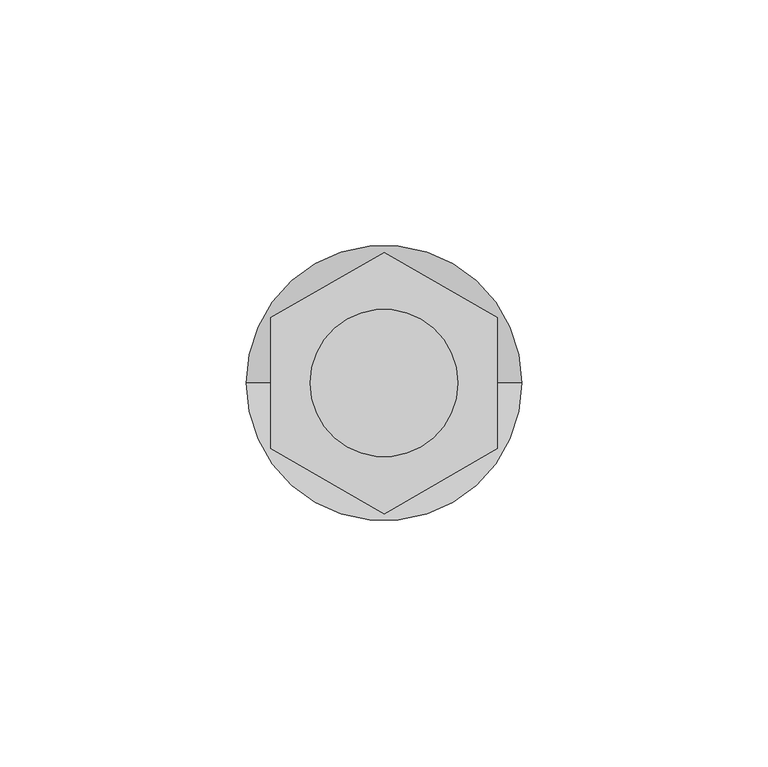
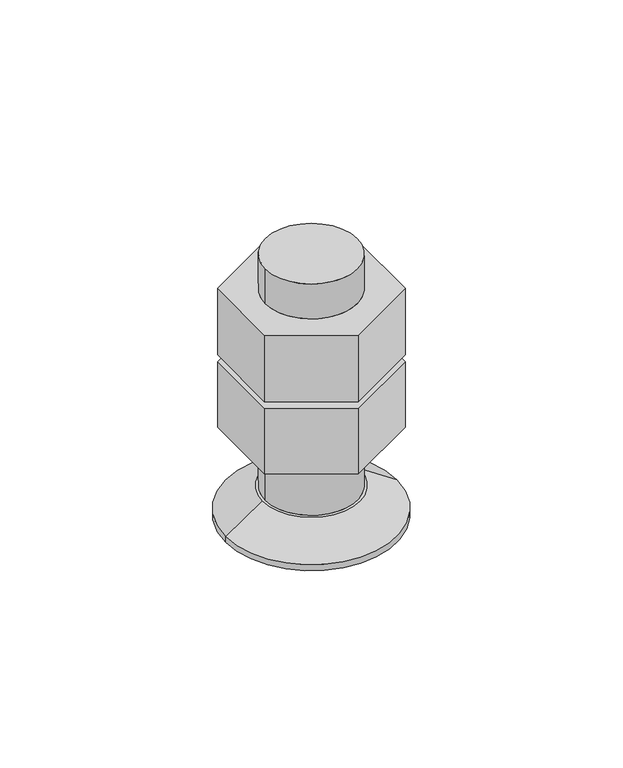
"""IFC4 building model written with IfcOpenShell, lengths in millimetres: fastener geometry, Bolt HPM-L : 30/L_mk."""

from ifc_helpers import new_model, si_unit, frame, origin, origin_with_axes, place, context, project, spatial, polyline, circle_curve, source, transform, mapped, element, save
from ifc_brep_helpers import plane_surface, cylinder_surface, revolved_surface, advanced_brep


def fastener_4f65ad77(model_context):
    return source(origin(), model_context, "Body", "AdvancedBrep", [
        advanced_brep(
        [(-23.0, 13.2790562, 22.7), (-23.0, -13.2790562, 22.7), (0.0, -26.5581124, 22.7), (23.0, -13.2790562, 22.7), (23.0, 13.2790562, 22.7), (0.0, 26.5581124, 22.7), (15.0, 0.0, 22.7), (-15.0, 0.0, 22.7), (-23.0, 13.2790562, 0.0), (0.0, 26.5581124, 0.0), (23.0, 13.2790562, 0.0), (23.0, -13.2790562, 0.0), (0.0, -26.5581124, 0.0), (-23.0, -13.2790562, 0.0), (-15.0, 0.0, 0.0), (15.0, 0.0, 0.0), (-15.0, 0.0, 60.0), (15.0, 0.0, 60.0), (15.0, 0.0, 25.0), (-15.0, 0.0, 25.0), (-15.0, 0.0, 48.0), (15.0, 0.0, 48.0), (-15.0, 0.0, -20.0), (15.0, 0.0, -20.0), (-23.0, 13.2790562, 48.0), (-23.0, -13.2790562, 48.0), (0.0, -26.5581124, 48.0), (23.0, -13.2790562, 48.0), (23.0, 13.2790562, 48.0), (0.0, 26.5581124, 48.0), (-23.0, 13.2790562, 25.0), (0.0, 26.5581124, 25.0), (23.0, 13.2790562, 25.0), (23.0, -13.2790562, 25.0), (0.0, -26.5581124, 25.0), (-23.0, -13.2790562, 25.0), (-28.0, 0.0, -30.0), (28.0, 0.0, -30.0), (28.0, 0.0, -28.0), (-28.0, 0.0, -28.0), (-16.0, 0.0, -20.0), (16.0, 0.0, -20.0)],
        [
            (0, 1),
            (1, 2),
            (2, 3),
            (3, 4),
            (4, 5),
            (5, 0),
            (6, 7, circle_curve(frame((0.0, 0.0, 22.7), z_axis=(0.0, 0.0, -1.0), x_axis=(1.0, 0.0, 0.0)), 15.0)),
            (7, 6, circle_curve(frame((0.0, 0.0, 22.7), z_axis=(0.0, 0.0, -1.0), x_axis=(1.0, 0.0, 0.0)), 15.0)),
            (8, 9),
            (9, 10),
            (10, 11),
            (11, 12),
            (12, 13),
            (13, 8),
            (14, 15, circle_curve(origin_with_axes(), 15.0)),
            (15, 14, circle_curve(origin_with_axes(), 15.0)),
            (0, 8),
            (13, 1),
            (12, 2),
            (11, 3),
            (10, 4),
            (9, 5),
            (16, 17, circle_curve(frame((0.0, 0.0, 60.0), z_axis=(0.0, 0.0, 1.0), x_axis=(1.0, 0.0, 0.0)), 15.0)),
            (17, 16, circle_curve(frame((0.0, 0.0, 60.0), z_axis=(0.0, 0.0, 1.0), x_axis=(1.0, 0.0, 0.0)), 15.0)),
            (6, 18),
            (18, 19, circle_curve(frame((0.0, 0.0, 25.0), z_axis=(0.0, 0.0, -1.0), x_axis=(1.0, 0.0, 0.0)), 15.0)),
            (19, 7),
            (16, 20),
            (20, 21, circle_curve(frame((0.0, 0.0, 48.0), z_axis=(0.0, 0.0, 1.0), x_axis=(1.0, 0.0, 0.0)), 15.0)),
            (21, 17),
            (14, 22),
            (22, 23, circle_curve(frame((0.0, 0.0, -20.0), z_axis=(0.0, 0.0, 1.0), x_axis=(1.0, 0.0, 0.0)), 15.0)),
            (23, 15),
            (19, 18, circle_curve(frame((0.0, 0.0, 25.0), z_axis=(0.0, 0.0, -1.0), x_axis=(1.0, 0.0, 0.0)), 15.0)),
            (21, 20, circle_curve(frame((0.0, 0.0, 48.0), z_axis=(0.0, 0.0, 1.0), x_axis=(1.0, 0.0, 0.0)), 15.0)),
            (23, 22, circle_curve(frame((0.0, 0.0, -20.0), z_axis=(0.0, 0.0, 1.0), x_axis=(1.0, 0.0, 0.0)), 15.0)),
            (24, 25),
            (25, 26),
            (26, 27),
            (27, 28),
            (28, 29),
            (29, 24),
            (30, 31),
            (31, 32),
            (32, 33),
            (33, 34),
            (34, 35),
            (35, 30),
            (24, 30),
            (35, 25),
            (34, 26),
            (33, 27),
            (32, 28),
            (31, 29),
            (36, 37, circle_curve(frame((0.0, 0.0, -30.0), z_axis=(0.0, 0.0, 1.0), x_axis=(1.0, 0.0, 0.0)), 28.0)),
            (37, 38),
            (38, 39, circle_curve(frame((0.0, 0.0, -28.0), z_axis=(0.0, 0.0, -1.0), x_axis=(1.0, 0.0, 0.0)), 28.0)),
            (39, 36),
            (37, 36, circle_curve(frame((0.0, 0.0, -30.0), z_axis=(0.0, 0.0, 1.0), x_axis=(1.0, 0.0, 0.0)), 28.0)),
            (39, 38, circle_curve(frame((0.0, 0.0, -28.0), z_axis=(0.0, 0.0, -1.0), x_axis=(1.0, 0.0, 0.0)), 28.0)),
            (40, 39),
            (38, 41),
            (41, 40, circle_curve(frame((0.0, 0.0, -20.0), z_axis=(0.0, 0.0, -1.0), x_axis=(1.0, 0.0, 0.0)), 16.0)),
            (40, 41, circle_curve(frame((0.0, 0.0, -20.0), z_axis=(0.0, 0.0, -1.0), x_axis=(-1.0, 0.0, 0.0)), 16.0)),
        ],
        [
            plane_surface(frame((-23.0, 13.2790562, 22.7), z_axis=(0.0, 0.0, 1.0), x_axis=(0.0, -1.0, 0.0))),
            plane_surface(frame((-23.0, 13.2790562, 0.0), z_axis=(0.0, 0.0, -1.0), x_axis=(0.0, 1.0, 0.0))),
            plane_surface(frame((-23.0, 13.2790562, 22.7), z_axis=(-1.0, 0.0, 0.0), x_axis=(0.0, 0.0, -1.0))),
            plane_surface(frame((-23.0, -13.2790562, 22.7), z_axis=(-0.4999999999999993, -0.8660254037844392, 0.0), x_axis=(0.0, 0.0, -1.0))),
            plane_surface(frame((0.0, -26.5581124, 22.7), z_axis=(0.5000000000000024, -0.8660254037844374, 0.0), x_axis=(0.0, 0.0, -1.0))),
            plane_surface(frame((23.0, -13.2790562, 22.7), z_axis=(1.0, 0.0, 0.0), x_axis=(0.0, 0.0, -1.0))),
            plane_surface(frame((23.0, 13.2790562, 22.7), z_axis=(0.4999999999999989, 0.8660254037844393, 0.0), x_axis=(0.0, 0.0, -1.0))),
            plane_surface(frame((0.0, 26.5581124, 22.7), z_axis=(-0.49999999999999895, 0.8660254037844393, 0.0), x_axis=(0.0, 0.0, -1.0))),
            plane_surface(frame((15.0, 0.0, 60.0), z_axis=(0.0, 0.0, 1.0), x_axis=(0.0, 1.0, 0.0))),
            cylinder_surface(frame((0.0, 0.0, -30.0), z_axis=(0.0, 0.0, 1.0), x_axis=(1.0, 0.0, 0.0)), 15.0),
            plane_surface(frame((-23.0, 13.2790562, 48.0), z_axis=(0.0, 0.0, 1.0), x_axis=(0.0, -1.0, 0.0))),
            plane_surface(frame((-23.0, 13.2790562, 25.0), z_axis=(0.0, 0.0, -1.0), x_axis=(0.0, 1.0, 0.0))),
            plane_surface(frame((-23.0, 13.2790562, 48.0), z_axis=(-1.0, 0.0, 0.0), x_axis=(0.0, 0.0, -1.0))),
            plane_surface(frame((-23.0, -13.2790562, 48.0), z_axis=(-0.4999999999999995, -0.866025403784439, 0.0), x_axis=(0.0, 0.0, -1.0))),
            plane_surface(frame((0.0, -26.5581124, 48.0), z_axis=(0.5000000000000024, -0.8660254037844373, 0.0), x_axis=(0.0, 0.0, -1.0))),
            plane_surface(frame((23.0, -13.2790562, 48.0), z_axis=(1.0, 0.0, 0.0), x_axis=(0.0, 0.0, -1.0))),
            plane_surface(frame((23.0, 13.2790562, 48.0), z_axis=(0.4999999999999991, 0.8660254037844393, 0.0), x_axis=(0.0, 0.0, -1.0))),
            plane_surface(frame((0.0, 26.5581124, 48.0), z_axis=(-0.49999999999999895, 0.8660254037844393, 0.0), x_axis=(0.0, 0.0, -1.0))),
            cylinder_surface(frame((0.0, 0.0, -30.0), z_axis=(0.0, 0.0, 1.0), x_axis=(1.0, 0.0, 0.0)), 28.0),
            revolved_surface(polyline([(-16.000000021428573, 0.0, -20.0), (-28.0, 0.0, -28.0)]), (0.0, 0.0, -9.3333333), (0.0, 0.0, -1.0)),
            plane_surface(frame((16.0, 0.0, -20.0), z_axis=(0.0, 0.0, 1.0), x_axis=(0.0, 1.0, 0.0))),
            plane_surface(frame((15.0, 0.0, -30.0), z_axis=(0.0, 0.0, -1.0), x_axis=(0.0, -1.0, 0.0))),
        ],
        [
            (0, [[1, 2, 3, 4, 5, 6], [7, 8]]),
            (1, [[9, 10, 11, 12, 13, 14], [15, 16]]),
            (2, [[-1, 17, -14, 18]]),
            (3, [[-2, -18, -13, 19]]),
            (4, [[-3, -19, -12, 20]]),
            (5, [[-4, -20, -11, 21]]),
            (6, [[-5, -21, -10, 22]]),
            (7, [[-6, -22, -9, -17]]),
            (8, [[23, 24]]),
            (9, [[-7, 25, 26, 27]]),
            (9, [[-23, 28, 29, 30]]),
            (9, [[-15, 31, 32, 33]]),
            (9, [[-8, -27, 34, -25]]),
            (9, [[-24, -30, 35, -28]]),
            (9, [[-16, -33, 36, -31]]),
            (10, [[37, 38, 39, 40, 41, 42], [-29, -35]]),
            (11, [[43, 44, 45, 46, 47, 48], [-26, -34]]),
            (12, [[-37, 49, -48, 50]]),
            (13, [[-38, -50, -47, 51]]),
            (14, [[-39, -51, -46, 52]]),
            (15, [[-40, -52, -45, 53]]),
            (16, [[-41, -53, -44, 54]]),
            (17, [[-42, -54, -43, -49]]),
            (18, [[55, 56, 57, 58]]),
            (18, [[59, -58, 60, -56]]),
            (19, [[61, -57, 62, 63]]),
            (19, [[-61, 64, -62, -60]]),
            (20, [[-63, -64], [-32, -36]]),
            (21, [[-59, -55]]),
        ],
    ),
    ])


if __name__ == "__main__":
    model = new_model("IFC4")
    model_context = context("Model", 3, world=origin())
    ifc_project = project(units=[si_unit("LENGTHUNIT", "METRE", prefix="MILLI")], contexts=[model_context])
    site = spatial("IfcSite", under=ifc_project)
    building = spatial("IfcBuilding", under=site)
    placement = place(None, origin())
    fastener_shape = fastener_4f65ad77(model_context)
    element("IfcFastener", 1, ObjectType="Bolt HPM-L : 30/L_mk", at=placement, inside=building, context=model_context, shape_type="MappedRepresentation", body=[
        mapped(fastener_shape, transform((0.0, 0.0, 0.0), x_axis=(1.0, 0.0, 0.0), y_axis=(0.0, 1.0, 0.0), z_axis=(0.0, 0.0, 1.0))),
    ])
    save(model, "model.ifc")

# Revit data of these elements
# Type "Bolt HPM-L : 30/L_mk"
#   Type Comments = "Mountingpart"
#   r3 = 15 mm
#   r2 = 28 mm
#   r1 = 16 mm
#   offset2 = 0 mm
#   l1 = 60 mm
#   Washer s = 8 mm
#   Washer Raduis2 = 32.5 mm
#   Washer Radius1 = 15.5 mm
#   Washer Diameter2 = 65 mm
#   Washer Diameter1 = 31 mm
#   T [instance default] = 45 mm
#   Offset1 [instance default] = 25 mm
#   Hexagonal nut m = 22.7 mm
#   l3 = 60 mm
#   l2 = 30 mm
#   hef = 20 mm
#   d3 = 30 mm
#   d1 = 32 mm
#   a = 90 mm
#   Hexagonal nut S1 = 23 mm
#   Hexagonal nut S = 46 mm
#   Material [instance default] = Metal - Steel - S355
#   Default Elevation = 0
# Element 1 (IfcFastener, "Bolt HPM-L : 30/L_mk")
#   Materials on its faces: "Metal - Steel - S355"
# Materials
#   "Metal - Steel - S355": class "Steel", colour RGB 247 247 247, transparency 0, Cost = 0
